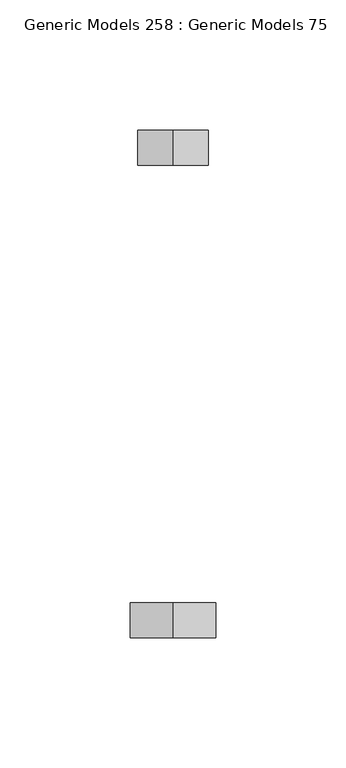
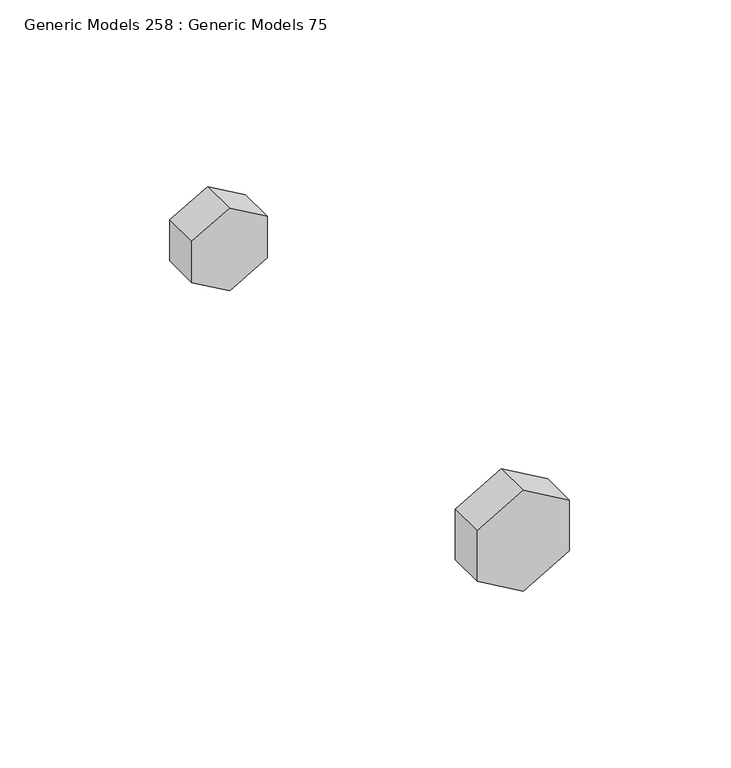
"""IFC4 building model written with IfcOpenShell, lengths in millimetres: proxy geometry, Generic Models 258 : Generic Models 75."""

from ifc_helpers import new_model, si_unit, frame, origin, place, context, project, spatial, polyline, outline, extrude, source, transform, mapped, element, save


def generic_models_258_generic_models_75_48cdfd2c(model_context):
    return source(origin(), model_context, "Body", "SweptSolid", [
        extrude(outline(polyline([(266693.030998, 32006.2068618), (266712.080998, 32006.2068618), (266721.605998, 31989.7090778), (266712.080998, 31973.2112939), (266693.030998, 31973.2112939), (266683.505998, 31989.7090778), (266693.030998, 32006.2068618)])), frame((0.0, 30676.7094112, 0.0), z_axis=(0.0, 1.0, 0.0), x_axis=(0.0, 0.0, 1.0)), (0.0, 0.0, 1.0), 13.49375),
        extrude(outline(polyline([(266710.1638403, 31976.2187024), (266694.5864965, 31976.2187024), (266686.7978246, 31989.7090778), (266694.5864965, 32003.1994532), (266710.1638403, 32003.1994532), (266717.9525121, 31989.7090778), (266710.1638403, 31976.2187024)])), frame((0.0, 30858.4781612, 0.0), z_axis=(0.0, 1.0, 0.0), x_axis=(0.0, 0.0, 1.0)), (0.0, 0.0, 1.0), 13.49375),
    ])


if __name__ == "__main__":
    model = new_model("IFC4")
    model_context = context("Model", 3, world=origin())
    ifc_project = project(units=[si_unit("LENGTHUNIT", "METRE", prefix="MILLI")], contexts=[model_context])
    site = spatial("IfcSite", under=ifc_project)
    building = spatial("IfcBuilding", under=site)
    placement = place(None, origin())
    generic_models_258_generic_models_75_shape = generic_models_258_generic_models_75_48cdfd2c(model_context)
    element("IfcBuildingElementProxy", 1, Name="Generic Models 258 : Generic Models 75", ObjectType="Generic Models 258 : Generic Models 75", at=placement, inside=building, context=model_context, shape_type="MappedRepresentation", body=[
        mapped(generic_models_258_generic_models_75_shape, transform((0.0, 0.0, 0.0), x_axis=(1.0, 0.0, 0.0), y_axis=(0.0, 1.0, 0.0), z_axis=(0.0, 0.0, 1.0))),
    ])
    save(model, "model.ifc")

# Revit data of these elements
# Element 1 (IfcBuildingElementProxy, "Generic Models 258 : Generic Models 75")
#   Materials on its faces: "3/4\" GALV. THRU BOLTS"
# Materials
#   "3/4\" GALV. THRU BOLTS": class "Generic", colour RGB 105 69 171, transparency 0, Cost = 0
